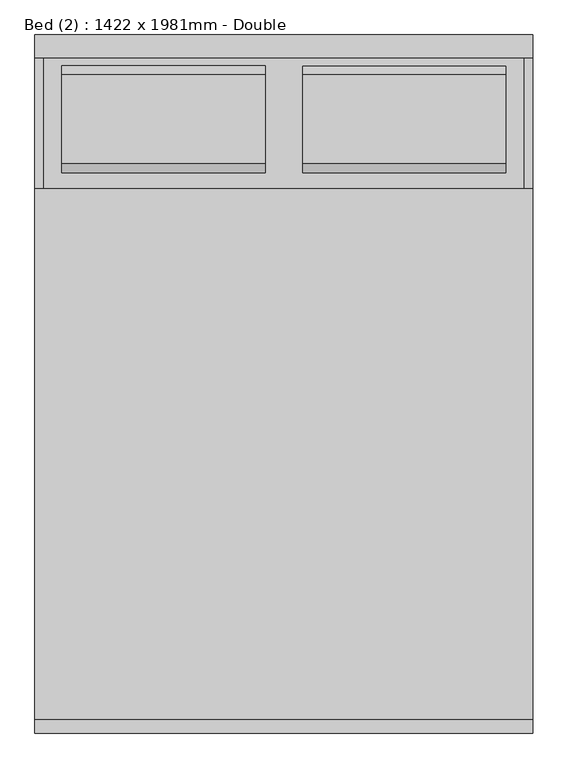
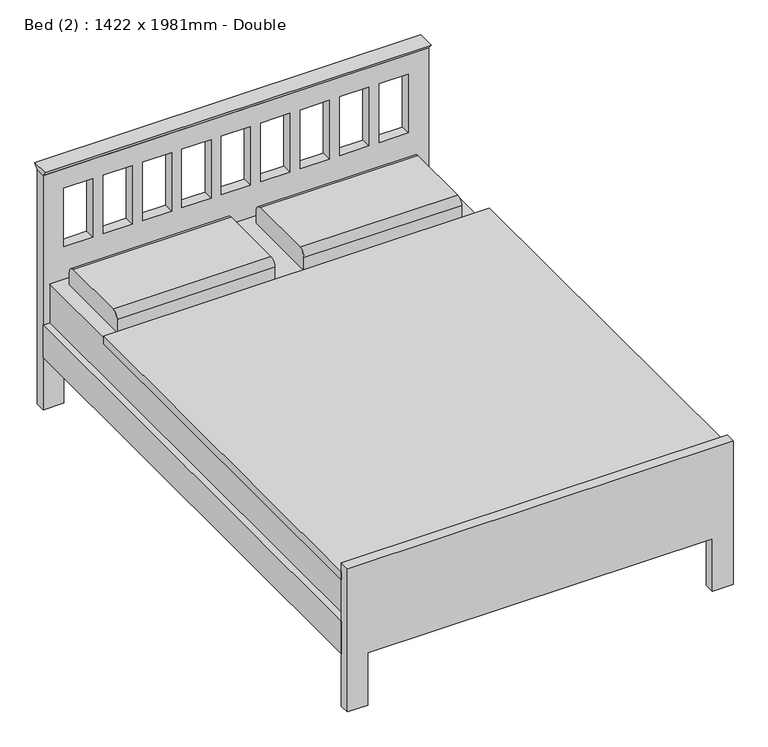
"""IFC4 building model written with IfcOpenShell, lengths in millimetres: furniture geometry, Bed (2) : 1422 x 1981mm - Double."""

from ifc_helpers import new_model, si_unit, point, frame, frame_2d, origin, place, context, project, spatial, polyline, circle_curve, trimmed, segment, composite_curve, outline, extrude, source, transform, mapped, element, save


def bed_2_1422_x_1981mm_double_43666e8e(model_context):
    return source(origin(), model_context, "Body", "SweptSolid", [
        extrude(outline(composite_curve([segment(polyline([(-380.0, 482.55), (-380.0, 533.35)]), True, "CONTINUOUS"), segment(trimmed(circle_curve(frame_2d((-354.6, 533.35)), 25.4), [point((-380.0, 533.35))], [point((-354.6, 558.75))], False, "CARTESIAN"), True, "CONTINUOUS"), segment(polyline([(-354.6, 558.75), (-100.6, 558.75)]), True, "CONTINUOUS"), segment(trimmed(circle_curve(frame_2d((-100.6, 533.35)), 25.4), [point((-100.6, 558.75))], [point((-75.2, 533.35))], False, "CARTESIAN"), True, "CONTINUOUS"), segment(polyline([(-75.2, 533.35), (-75.2, 482.55), (-380.0, 482.55)]), True, "CONTINUOUS")], self_intersect=False)), frame((34.5722222, 0.0, 0.0), z_axis=(1.0, 0.0, 0.0), x_axis=(0.0, 1.0, 0.0)), (0.0, 0.0, 1.0), 581.3777778),
        extrude(outline(polyline([(-38.1, 914.4), (-51.9545455, 933.45), (13.8545455, 933.45), (0.0, 914.4), (-38.1, 914.4)])), frame((-730.0365546, 0.0, 0.0), z_axis=(1.0, 0.0, 0.0), x_axis=(0.0, 1.0, 0.0)), (0.0, 0.0, 1.0), 1422.4533613),
        extrude(outline(composite_curve([segment(polyline([(-379.4173224, 482.6), (-379.4173224, 533.4)]), True, "CONTINUOUS"), segment(trimmed(circle_curve(frame_2d((-354.0173224, 533.4)), 25.4), [point((-379.4173224, 533.4))], [point((-354.0173224, 558.8))], False, "CARTESIAN"), True, "CONTINUOUS"), segment(polyline([(-354.0173224, 558.8), (-100.0173224, 558.8)]), True, "CONTINUOUS"), segment(trimmed(circle_curve(frame_2d((-100.0173224, 533.4)), 25.4), [point((-100.0173224, 558.8))], [point((-74.6173224, 533.4))], False, "CARTESIAN"), True, "CONTINUOUS"), segment(polyline([(-74.6173224, 533.4), (-74.6173224, 482.6), (-379.4173224, 482.6)]), True, "CONTINUOUS")], self_intersect=False)), frame((-654.05, 0.0, 0.0), z_axis=(1.0, 0.0, 0.0), x_axis=(0.0, 1.0, 0.0)), (0.0, 0.0, 1.0), 581.3777778),
        extrude(outline(polyline([(666.75, -38.1), (666.75, -1943.1), (-704.85, -1943.1), (-704.85, -38.1), (666.75, -38.1)])), frame((0.0, 0.0, 203.2), z_axis=(0.0, 0.0, 1.0), x_axis=(1.0, 0.0, 0.0)), (0.0, 0.0, 1.0), 279.4),
        extrude(outline(polyline([(666.75, -1943.1), (666.75, -38.1), (692.15, -38.1), (692.15, -1943.1), (666.75, -1943.1)])), frame((0.0, 0.0, 203.0994861), z_axis=(0.0, 0.0, 1.0), x_axis=(1.0, 0.0, 0.0)), (0.0, 0.0, 1.0), 127.0),
        extrude(outline(polyline([(-730.25, -1943.1), (-730.25, -38.1), (-704.85, -38.1), (-704.85, -1943.1), (-730.25, -1943.1)])), frame((0.0, 0.0, 203.5755296), z_axis=(0.0, 0.0, 1.0), x_axis=(1.0, 0.0, 0.0)), (0.0, 0.0, 1.0), 127.0),
        extrude(outline(polyline([(0.0, -654.05), (203.2, -654.05), (203.2, 615.95), (0.0, 615.95), (0.0, 692.15), (558.8, 692.15), (558.8, -730.25), (0.0, -730.25), (0.0, -654.05)])), frame((0.0, -1981.2, 0.0), z_axis=(0.0, 1.0, 0.0), x_axis=(0.0, 0.0, 1.0)), (0.0, 0.0, 1.0), 38.1),
        extrude(outline(polyline([(914.4, 692.4168067), (914.4, -730.0365546), (0.0, -730.0365546), (0.0, -654.05), (203.2, -654.05), (203.2, 615.95), (0.0, 615.95), (0.0, 692.4168067), (914.4, 692.4168067)]), holes=[polyline([(838.2, -546.8055556), (609.6, -546.8055556), (609.6, -654.05), (838.2, -654.05), (838.2, -546.8055556)]), polyline([(838.2, -401.4611111), (609.6, -401.4611111), (609.6, -508.7055556), (838.2, -508.7055556), (838.2, -401.4611111)]), polyline([(838.2, -256.1166667), (609.6, -256.1166667), (609.6, -363.3611111), (838.2, -363.3611111), (838.2, -256.1166667)]), polyline([(838.2, -110.7722222), (609.6, -110.7722222), (609.6, -218.0166667), (838.2, -218.0166667), (838.2, -110.7722222)]), polyline([(838.2, 179.9166667), (609.6, 179.9166667), (609.6, 72.6722222), (838.2, 72.6722222), (838.2, 179.9166667)]), polyline([(838.2, 325.2611111), (609.6, 325.2611111), (609.6, 218.0166667), (838.2, 218.0166667), (838.2, 325.2611111)]), polyline([(838.2, 470.6055556), (609.6, 470.6055556), (609.6, 363.3611111), (838.2, 363.3611111), (838.2, 470.6055556)]), polyline([(838.2, 615.95), (609.6, 615.95), (609.6, 508.7055556), (838.2, 508.7055556), (838.2, 615.95)]), polyline([(838.2, 34.5722222), (609.6, 34.5722222), (609.6, -72.6722222), (838.2, -72.6722222), (838.2, 34.5722222)])]), frame((0.0, -38.1, 0.0), z_axis=(0.0, 1.0, 0.0), x_axis=(0.0, 0.0, 1.0)), (0.0, 0.0, 1.0), 38.1),
        extrude(outline(polyline([(-730.25, -1943.1), (-730.25, -425.390138), (692.15, -425.390138), (692.15, -1943.1), (-730.25, -1943.1)])), frame((0.0, 0.0, 492.6), z_axis=(0.0, 0.0, 1.0), x_axis=(1.0, 0.0, 0.0)), (0.0, 0.0, 1.0), 31.2),
    ])


if __name__ == "__main__":
    model = new_model("IFC4")
    model_context = context("Model", 3, world=origin())
    ifc_project = project(units=[si_unit("LENGTHUNIT", "METRE", prefix="MILLI")], contexts=[model_context])
    site = spatial("IfcSite", under=ifc_project)
    building = spatial("IfcBuilding", under=site)
    placement = place(None, origin())
    bed_2_1422_x_1981mm_double_shape = bed_2_1422_x_1981mm_double_43666e8e(model_context)
    element("IfcFurniture", 1, ObjectType="Bed (2) : 1422 x 1981mm - Double", at=placement, inside=building, context=model_context, shape_type="MappedRepresentation", body=[
        mapped(bed_2_1422_x_1981mm_double_shape, transform((0.0, 0.0, 0.0), x_axis=(1.0, 0.0, 0.0), y_axis=(0.0, 1.0, 0.0), z_axis=(0.0, 0.0, 1.0))),
    ])
    save(model, "model.ifc")

# Revit data of these elements
# Type "Bed (2) : 1422 x 1981mm - Double"
#   Keynote = "N"
#   Length = 1981.2 mm
#   Width = 1422.4 mm
#   Material Frame = Wood - Birch
#   Material Mattress = Textile - White
# Element 1 (IfcFurniture, "Bed (2) : 1422 x 1981mm - Double")
#   Materials on its faces: "Wood - Birch", "Textile - White"
# Materials
#   "Wood - Birch": class "Wood", colour RGB 224 178 126, transparency 0
#   "Textile - White": class "Fabric", colour RGB 247 247 239, transparency 0
